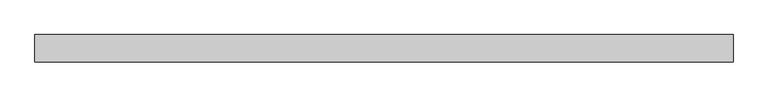
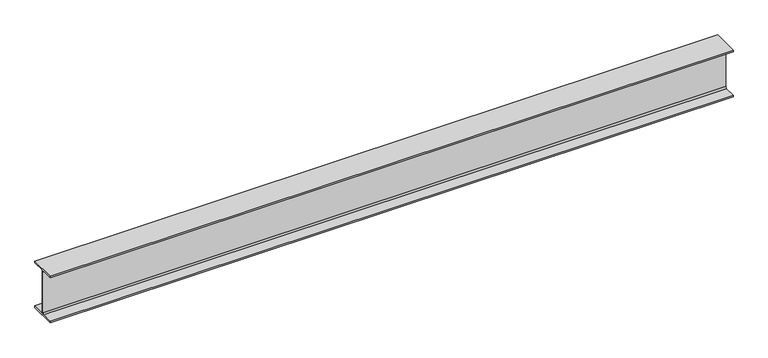
"""IFC4 building model written with IfcOpenShell, lengths in millimetres: beam geometry, Old_Steel Beam_H-KSD3502 : H_SB_ASB_H-300×300x10x15."""

from ifc_helpers import new_model, si_unit, point, frame, frame_2d, origin, place, context, project, spatial, polyline, circle_curve, trimmed, segment, composite_curve, outline, extrude, source, transform, mapped, element, save


def beam_36f1b8b6(model_context):
    return source(origin(), model_context, "Body", "SweptSolid", [
        extrude(outline(composite_curve([segment(polyline([(82.5, -141.5), (82.5, -151.7), (-82.5, -151.7), (-82.5, -141.5), (-11.9, -141.5)]), True, "CONTINUOUS"), segment(trimmed(circle_curve(frame_2d((-11.9, -132.6)), 8.9), [point((-11.9, -141.5))], [point((-3.0, -132.6))], True, "CARTESIAN"), True, "CONTINUOUS"), segment(polyline([(-3.0, -132.6), (-3.0, 132.6)]), True, "CONTINUOUS"), segment(trimmed(circle_curve(frame_2d((-11.9, 132.6)), 8.9), [point((-3.0, 132.6))], [point((-11.9, 141.5))], True, "CARTESIAN"), True, "CONTINUOUS"), segment(polyline([(-11.9, 141.5), (-82.5, 141.5), (-82.5, 151.7), (82.5, 151.7), (82.5, 141.5), (11.9, 141.5)]), True, "CONTINUOUS"), segment(trimmed(circle_curve(frame_2d((11.9, 132.6)), 8.9), [point((11.9, 141.5))], [point((3.0, 132.6))], True, "CARTESIAN"), True, "CONTINUOUS"), segment(polyline([(3.0, 132.6), (3.0, -132.6)]), True, "CONTINUOUS"), segment(trimmed(circle_curve(frame_2d((11.9, -132.6)), 8.9), [point((3.0, -132.6))], [point((11.9, -141.5))], True, "CARTESIAN"), True, "CONTINUOUS"), segment(polyline([(11.9, -141.5), (82.5, -141.5)]), True, "CONTINUOUS")], self_intersect=False)), frame((-2849.2330406, 0.0, 0.0), z_axis=(1.0, 0.0, 0.0), x_axis=(0.0, 1.0, 0.0)), (0.0, 0.0, 1.0), 4213.4660812),
    ])


if __name__ == "__main__":
    model = new_model("IFC4")
    model_context = context("Model", 3, world=origin())
    ifc_project = project(units=[si_unit("LENGTHUNIT", "METRE", prefix="MILLI")], contexts=[model_context])
    site = spatial("IfcSite", under=ifc_project)
    building = spatial("IfcBuilding", under=site)
    placement = place(None, origin())
    beam_shape = beam_36f1b8b6(model_context)
    element("IfcBeam", 1, ObjectType="Old_Steel Beam_H-KSD3502 : H_SB_ASB_H-300×300x10x15", at=placement, inside=building, context=model_context, shape_type="MappedRepresentation", body=[
        mapped(beam_shape, transform((0.0, 0.0, 0.0), x_axis=(1.0, 0.0, 0.0), y_axis=(0.0, 1.0, 0.0), z_axis=(0.0, 0.0, 1.0))),
    ])
    save(model, "model.ifc")

# Revit data of these elements
# Type "Old_Steel Beam_H-KSD3502 : H_SB_ASB_H-300×300x10x15"
#   Width = 30.0 cm
#   Web Thickness = 1.0 cm
#   Web Fillet = 1.8 cm
#   Warping Constant = 1370670.0 cm⁶
#   Torsional Moment of Inertia = 77.00 cm⁴
#   Torsional Modulus = 1.0 cm³
#   Section Area = 119.8 cm²
#   Plastic Modulus weak axis = 684.0 cm³
#   Plastic Modulus strong axis = 1500.0 cm³
#   Perimeter = 1.75 m²/m
#   Nominal Weight = 94.00 kgf/m
#   Moment of Inertia weak axis = 6750.00 cm⁴
#   Moment of Inertia strong axis = 20400.00 cm⁴
#   Height = 30.0 cm
#   Flange Thickness = 1.5 cm
#   Elastic Modulus weak axis = 450.0 cm³
#   Elastic Modulus strong axis = 1360.0 cm³
#   Centroid Vertical = 15.0 cm
#   Centroid Horizontal = 15.0 cm
#   Length [instance default] = 1.5240 m
#   Structural Material [instance default] = Steel, 45-345
#   Assembly Code = ""
# Element 1 (IfcBeam, "Old_Steel Beam_H-KSD3502 : H_SB_ASB_H-300×300x10x15")
#   Structural Material = none
# Materials
#   "Steel, 45-345": class "Metal", colour RGB 189 187 185, transparency 0, Description = "Steel 345 MPa", Cost = 0
